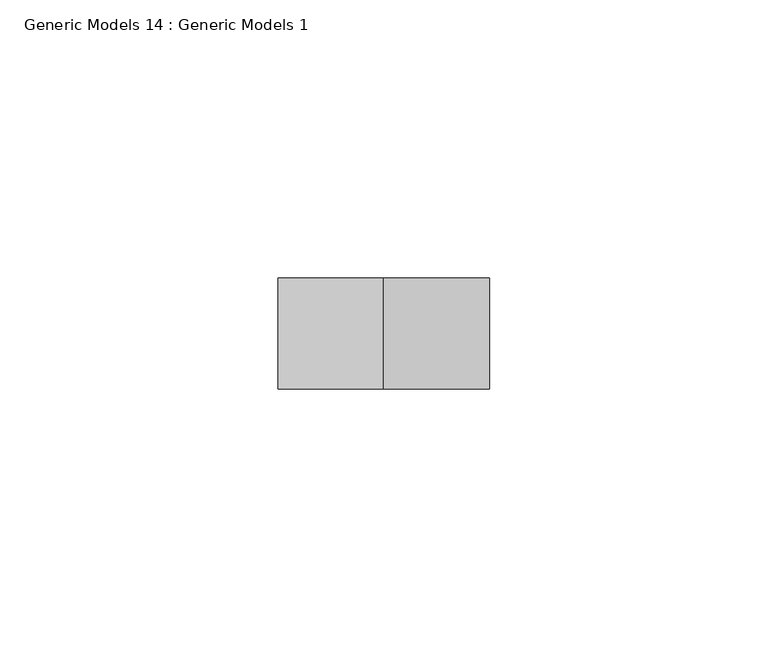
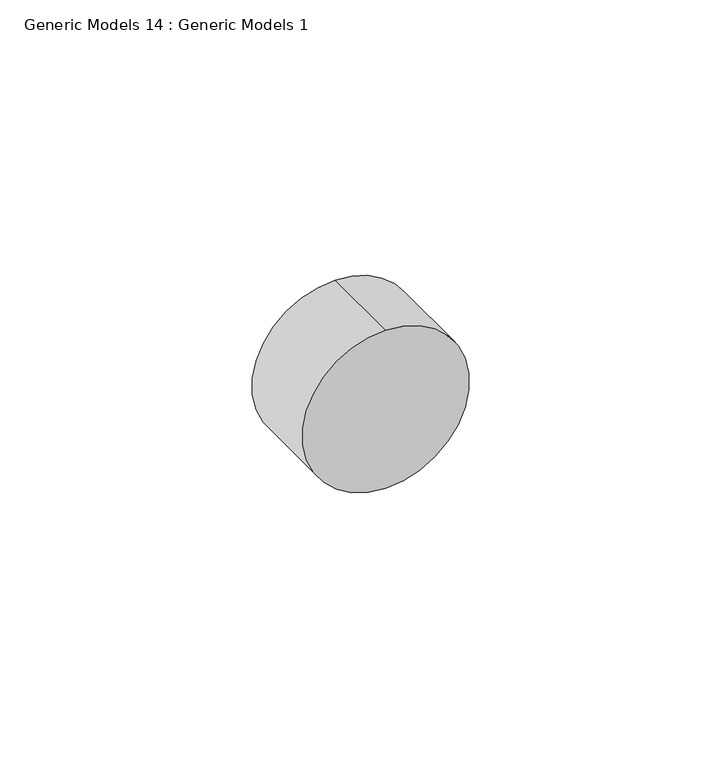
"""IFC4 building model written with IfcOpenShell, lengths in millimetres: proxy geometry, Generic Models 14 : Generic Models 1."""

from ifc_helpers import new_model, si_unit, point, frame, frame_2d, origin, place, context, project, spatial, circle_curve, trimmed, segment, composite_curve, outline, extrude, source, transform, mapped, element, save


def generic_models_14_generic_models_1_482cc507(model_context):
    return source(origin(), model_context, "Body", "SweptSolid", [
        extrude(outline(composite_curve([segment(trimmed(circle_curve(frame_2d((39943.2190778, 10206.2283642)), 19.1), [point((39924.1190778, 10206.2283642))], [point((39962.3190778, 10206.2283642))], False, "CARTESIAN"), True, "CONTINUOUS"), segment(trimmed(circle_curve(frame_2d((39943.2190778, 10206.2283642)), 19.1), [point((39962.3190778, 10206.2283642))], [point((39924.1190778, 10206.2283642))], False, "CARTESIAN"), True, "CONTINUOUS")], self_intersect=False)), frame((0.0, 2006.3413727, 0.0), z_axis=(0.0, 1.0, 0.0), x_axis=(0.0, 0.0, 1.0)), (0.0, 0.0, 1.0), 19.9567516),
    ])


if __name__ == "__main__":
    model = new_model("IFC4")
    model_context = context("Model", 3, world=origin())
    ifc_project = project(units=[si_unit("LENGTHUNIT", "METRE", prefix="MILLI")], contexts=[model_context])
    site = spatial("IfcSite", under=ifc_project)
    building = spatial("IfcBuilding", under=site)
    placement = place(None, origin())
    generic_models_14_generic_models_1_shape = generic_models_14_generic_models_1_482cc507(model_context)
    element("IfcBuildingElementProxy", 1, Name="Generic Models 14 : Generic Models 1", ObjectType="Generic Models 14 : Generic Models 1", at=placement, inside=building, context=model_context, shape_type="MappedRepresentation", body=[
        mapped(generic_models_14_generic_models_1_shape, transform((0.0, 0.0, 0.0), x_axis=(1.0, 0.0, 0.0), y_axis=(0.0, 1.0, 0.0), z_axis=(0.0, 0.0, 1.0))),
    ])
    save(model, "model.ifc")
